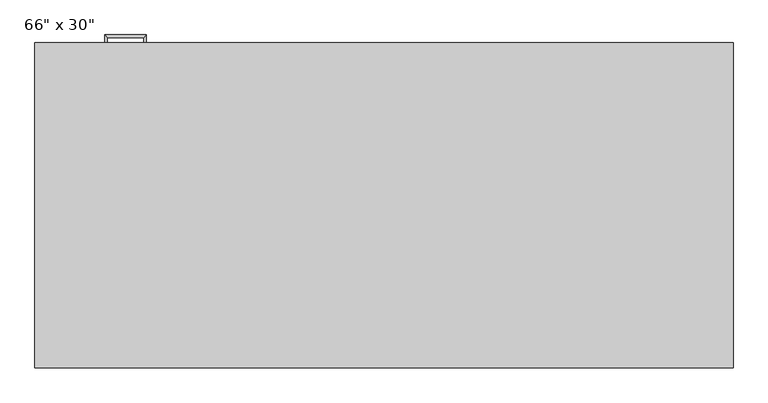
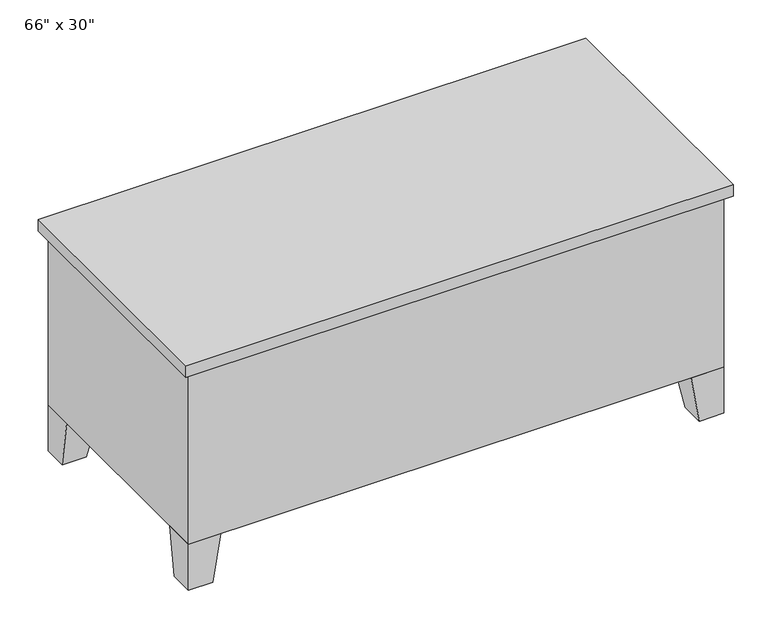
"""IFC4 building model written with IfcOpenShell, lengths in millimetres: furniture geometry."""

import ifcopenshell
import ifcopenshell.guid

model = None  # the IFC model being written
_history = None  # IfcOwnerHistory: only IFC2X3 demands one
_inside = {}  # id of a spatial element -> (the spatial element, [elements in it])
_under = {}  # id of a project, library or spatial element -> (it, [spatial elements below it])
_declared = {}  # id of a project -> (the project, [libraries it declares])
_typed = {}  # id of a type object -> (the type object, [elements of that type])
_made_of = {}  # id of a material, layer set ... -> (it, [elements and type objects made of it])


def new_model(schema):
    """Start an empty IFC model of exactly this schema.

    Asked for "IFC4X3", IfcOpenShell would pick the latest addendum, in which some entities
    have other attributes; the version numbers below select the first issue.
    IFC2X3 requires an IfcOwnerHistory on every rooted entity: one is made here for all.
    """
    global model, _history
    if schema == "IFC4X3":
        model = ifcopenshell.file(schema_version=(4, 3, 0, 0))
    else:
        model = ifcopenshell.file(schema=schema)
    _inside.clear()
    _under.clear()
    _declared.clear()
    _typed.clear()
    _made_of.clear()
    _history = None
    if model.schema == "IFC2X3":
        org = make("IfcOrganization", Name="unknown")
        user = make(
            "IfcPersonAndOrganization",
            ThePerson=make("IfcPerson", FamilyName="unknown"),
            TheOrganization=org,
        )
        app = make(
            "IfcApplication",
            ApplicationDeveloper=org,
            Version="unknown",
            ApplicationFullName="unknown",
            ApplicationIdentifier="unknown",
        )
        _history = make(
            "IfcOwnerHistory",
            OwningUser=user,
            OwningApplication=app,
            ChangeAction="ADDED",
            CreationDate=0,
        )
    return model


def make(cls, **values):
    """One entity of the class cls with the attributes given. An attribute that is None is left unset."""
    return model.create_entity(
        cls, **{name: value for name, value in values.items() if value is not None}
    )


def rooted(cls, **values):
    """An entity with a GlobalId (a new one), such as an element, a storey or a relation."""
    return make(cls, GlobalId=ifcopenshell.guid.new(), OwnerHistory=_history, **values)


def si_unit(unit_type, name, prefix=None):
    """IfcSIUnit, for example si_unit("LENGTHUNIT", "METRE", prefix="MILLI")."""
    return make("IfcSIUnit", UnitType=unit_type, Prefix=prefix, Name=name)


def assignment(units):
    """IfcUnitAssignment: the units of a project."""
    return None if units is None else make("IfcUnitAssignment", Units=units)


def point(xyz):
    """IfcCartesianPoint."""
    return None if xyz is None else make("IfcCartesianPoint", Coordinates=xyz)


def direction(xyz):
    """IfcDirection."""
    return None if xyz is None else make("IfcDirection", DirectionRatios=xyz)


def frame(location, z_axis=None, x_axis=None):
    """IfcAxis2Placement3D, a coordinate frame: its origin and axes. An axis left out is left unset."""
    return make(
        "IfcAxis2Placement3D",
        Location=point(location),
        Axis=direction(z_axis),
        RefDirection=direction(x_axis),
    )


def origin():
    """The frame at (0, 0, 0) with its axes left unset."""
    return frame((0.0, 0.0, 0.0))


def place(relative_to, where):
    """IfcLocalPlacement: puts the frame where relative to a parent placement (None: the world)."""
    return make(
        "IfcLocalPlacement", PlacementRelTo=relative_to, RelativePlacement=where
    )


def context(
    kind, dimensions, precision=None, world=None, true_north=None, identifier=None
):
    """IfcGeometricRepresentationContext, for example the 3D "Model" context."""
    return make(
        "IfcGeometricRepresentationContext",
        ContextIdentifier=identifier,
        ContextType=kind,
        CoordinateSpaceDimension=dimensions,
        Precision=precision,
        WorldCoordinateSystem=world,
        TrueNorth=true_north,
    )


def project(units=None, contexts=None):
    """IfcProject with its units and contexts."""
    return rooted(
        "IfcProject",
        Name="project",
        RepresentationContexts=contexts,
        UnitsInContext=assignment(units),
    )


def spatial(cls, under=None, at=None, **own):
    """A site, building, storey or space (cls), placed at a placement, below another one or the project."""
    s = rooted(cls, ObjectPlacement=at, **own)
    if under is not None:
        _under.setdefault(under.id(), (under, []))[1].append(s)
    return s


def polyline(points):
    """IfcPolyline through the points."""
    return make("IfcPolyline", Points=[point(p) for p in points])


def outline(outer, holes=None, kind="AREA"):
    """IfcArbitraryClosedProfileDef: a profile drawn as a closed curve; with holes, ...WithVoids."""
    if holes is None:
        return make("IfcArbitraryClosedProfileDef", ProfileType=kind, OuterCurve=outer)
    return make(
        "IfcArbitraryProfileDefWithVoids",
        ProfileType=kind,
        OuterCurve=outer,
        InnerCurves=holes,
    )


def extrude(swept, where, along, depth):
    """IfcExtrudedAreaSolid: the profile swept, set in the frame where, extruded along a direction by depth."""
    return make(
        "IfcExtrudedAreaSolid",
        SweptArea=swept,
        Position=where,
        ExtrudedDirection=direction(along),
        Depth=depth,
    )


def faces_of(points, faces, orient=None, outer=None):
    """IfcFace entities. A face is a list of loops; a loop is a list of indices into points, from 0.

    orient and outer hold one flag for each loop. By default every Orientation is true, the
    first loop of a face is its IfcFaceOuterBound and the others are IfcFaceBound.
    """
    made = []
    for i, loops in enumerate(faces):
        bounds = []
        for j, loop in enumerate(loops):
            is_outer = j == 0 if outer is None else outer[i][j]
            bounds.append(
                make(
                    "IfcFaceOuterBound" if is_outer else "IfcFaceBound",
                    Bound=make("IfcPolyLoop", Polygon=[points[k] for k in loop]),
                    Orientation=True if orient is None else orient[i][j],
                )
            )
        made.append(make("IfcFace", Bounds=bounds))
    return made


def faceted_brep(points, faces, orient=None, outer=None, voids=None):
    """IfcFacetedBrep: a solid bounded by flat faces; with voids (closed shells), ...WithVoids."""
    shared = [point(p) for p in points]
    hull = make("IfcClosedShell", CfsFaces=faces_of(shared, faces, orient, outer))
    if voids is None:
        return make("IfcFacetedBrep", Outer=hull)
    return make(
        "IfcFacetedBrepWithVoids",
        Outer=hull,
        Voids=[
            make(cls, CfsFaces=faces_of(shared, fs, o, b)) for cls, fs, o, b in voids
        ],
    )


def shape(context_of_items, identifier, shape_type, items):
    """IfcShapeRepresentation: the items that make up one representation, for example the "Body"."""
    return make(
        "IfcShapeRepresentation",
        ContextOfItems=context_of_items,
        RepresentationIdentifier=identifier,
        RepresentationType=shape_type,
        Items=items,
    )


def source(mapping_origin, context_of_items, identifier, shape_type, items):
    """IfcRepresentationMap: a shape defined once, which mapped items show again and again."""
    return make(
        "IfcRepresentationMap",
        MappingOrigin=mapping_origin,
        MappedRepresentation=shape(context_of_items, identifier, shape_type, items),
    )


def transform(
    local_origin,
    x_axis=None,
    y_axis=None,
    z_axis=None,
    scale=None,
    scale2=None,
    scale3=None,
    uniform=True,
):
    """IfcCartesianTransformationOperator3D, or its non-uniform kind. x_axis, y_axis, z_axis: its Axis1, 2, 3."""
    if uniform:
        return make(
            "IfcCartesianTransformationOperator3D",
            Axis1=direction(x_axis),
            Axis2=direction(y_axis),
            LocalOrigin=point(local_origin),
            Scale=scale,
            Axis3=direction(z_axis),
        )
    return make(
        "IfcCartesianTransformationOperator3DnonUniform",
        Axis1=direction(x_axis),
        Axis2=direction(y_axis),
        LocalOrigin=point(local_origin),
        Scale=scale,
        Axis3=direction(z_axis),
        Scale2=scale2,
        Scale3=scale3,
    )


def mapped(mapping_source, mapping_target):
    """IfcMappedItem: shows the shape of a source again, moved by a transform."""
    return make(
        "IfcMappedItem", MappingSource=mapping_source, MappingTarget=mapping_target
    )


def made_of(thing, what):
    """Note that an element or type object is made of a material, layer set ...; save() writes the relation."""
    if what is not None:
        _made_of.setdefault(what.id(), (what, []))[1].append(thing)
    return thing


def element(
    cls,
    number,
    at=None,
    inside=None,
    cuts=None,
    type_object=None,
    material=None,
    context=None,
    identifier="Body",
    shape_type=None,
    held_by="IfcProductDefinitionShape",
    body=None,
    shapes=None,
    **own,
):
    """One element of the class cls, such as IfcWall. Its Tag is "e" and its number.

    at: its placement. inside: the storey or other place that contains it. cuts: it is an
    opening in that element (IfcRelVoidsElement). A single representation is given by context,
    identifier, shape_type and body (its items); several are given by shapes. held_by: the class
    of the entity that holds the representations. save() writes the other relations.
    """
    e = rooted(cls, Tag="e%d" % number, ObjectPlacement=at, **own)
    if body is not None:
        shapes = [shape(context, identifier, shape_type, body)]
    if shapes is not None:
        e.Representation = make(held_by, Representations=shapes)
    if inside is not None:
        _inside.setdefault(inside.id(), (inside, []))[1].append(e)
    if cuts is not None:
        rooted(
            "IfcRelVoidsElement", RelatingBuildingElement=cuts, RelatedOpeningElement=e
        )
    if type_object is not None:
        _typed.setdefault(type_object.id(), (type_object, []))[1].append(e)
    return made_of(e, material)


def aggregate(whole, parts):
    """IfcRelAggregates: a whole, such as a stair, and the parts it consists of."""
    return rooted("IfcRelAggregates", RelatingObject=whole, RelatedObjects=parts)


def save(model, path):
    """Write the relations noted so far, then the file.

    IfcRelAggregates (storeys below a building ...), IfcRelContainedInSpatialStructure (elements
    in a storey), IfcRelDefinesByType, IfcRelAssociatesMaterial and IfcRelDeclares: one each for
    every whole, place, type object, material and project.
    """
    for whole, parts in _under.values():
        aggregate(whole, parts)
    for where, things in _inside.values():
        rooted(
            "IfcRelContainedInSpatialStructure",
            RelatedElements=things,
            RelatingStructure=where,
        )
    for kind, things in _typed.values():
        rooted("IfcRelDefinesByType", RelatedObjects=things, RelatingType=kind)
    for what, things in _made_of.values():
        rooted("IfcRelAssociatesMaterial", RelatedObjects=things, RelatingMaterial=what)
    for by, libraries in _declared.values():
        rooted("IfcRelDeclares", RelatingContext=by, RelatedDefinitions=libraries)
    model.write(path)


def furniture_388a94df(model_context):
    return source(origin(), model_context, "Body", "SolidModel", [
        faceted_brep([(406.4, 762.0, 723.9), (0.0, 762.0, 723.9), (0.0, 0.0, 723.9), (1676.4, 0.0, 723.9), (1676.4, 762.0, 723.9), (1422.4, 762.0, 723.9), (1422.4, 50.8, 723.9), (406.4, 50.8, 723.9), (406.4, 762.0, 152.4), (406.4, 50.8, 152.4), (1422.4, 50.8, 152.4), (1422.4, 762.0, 152.4), (1676.4, 762.0, 152.4), (1676.4, 0.0, 152.4), (0.0, 0.0, 152.4), (0.0, 762.0, 152.4), (1441.45, 762.0, 171.45), (1657.35, 762.0, 171.45), (1657.35, 762.0, 704.85), (1441.45, 762.0, 704.85), (1441.45, 50.8, 171.45), (1441.45, 50.8, 704.85), (1657.35, 50.8, 704.85), (1657.35, 50.8, 171.45)], [[[0, 1, 2, 3, 4, 5, 6, 7]], [[8, 9, 10, 11, 12, 13, 14, 15]], [[1, 0, 8, 15]], [[2, 1, 15, 14]], [[3, 2, 14, 13]], [[4, 3, 13, 12]], [[5, 4, 12, 11], [16, 17, 18, 19]], [[6, 5, 11, 10]], [[7, 6, 10, 9]], [[0, 7, 9, 8]], [[20, 21, 22, 23]], [[20, 23, 17, 16]], [[23, 22, 18, 17]], [[22, 21, 19, 18]], [[21, 20, 16, 19]]]),
        extrude(outline(polyline([(387.35, 762.0), (19.05, 762.0), (19.05, 774.7), (387.35, 774.7), (387.35, 762.0)])), frame((0.0, 0.0, 603.25), z_axis=(0.0, 0.0, 1.0), x_axis=(1.0, 0.0, 0.0)), (0.0, 0.0, 1.0), 101.6),
        extrude(outline(polyline([(387.35, 762.0), (19.05, 762.0), (19.05, 774.7), (387.35, 774.7), (387.35, 762.0)])), frame((0.0, 0.0, 171.45), z_axis=(0.0, 0.0, 1.0), x_axis=(1.0, 0.0, 0.0)), (0.0, 0.0, 1.0), 171.45),
        extrude(outline(polyline([(387.35, 762.0), (19.05, 762.0), (19.05, 774.7), (387.35, 774.7), (387.35, 762.0)])), frame((0.0, 0.0, 482.6), z_axis=(0.0, 0.0, 1.0), x_axis=(1.0, 0.0, 0.0)), (0.0, 0.0, 1.0), 101.6),
        extrude(outline(polyline([(387.35, 762.0), (19.05, 762.0), (19.05, 774.7), (387.35, 774.7), (387.35, 762.0)])), frame((0.0, 0.0, 361.95), z_axis=(0.0, 0.0, 1.0), x_axis=(1.0, 0.0, 0.0)), (0.0, 0.0, 1.0), 101.6),
        faceted_brep([(1574.8, 762.0, 152.4), (1574.8, 660.4, 152.4), (1676.4, 660.4, 152.4), (1676.4, 762.0, 152.4), (1600.2, 762.0, 0.0), (1676.4, 762.0, 0.0), (1676.4, 685.8, 0.0), (1600.2, 685.8, 0.0)], [[[0, 1, 2, 3]], [[4, 5, 6, 7]], [[4, 7, 1, 0]], [[7, 6, 2, 1]], [[6, 5, 3, 2]], [[5, 4, 0, 3]]]),
        faceted_brep([(1574.8, 0.0, 152.4), (1676.4, 0.0, 152.4), (1676.4, 101.6, 152.4), (1574.8, 101.6, 152.4), (1600.2, 0.0, 0.0), (1600.2, 76.2, 0.0), (1676.4, 76.2, 0.0), (1676.4, 0.0, 0.0)], [[[0, 1, 2, 3]], [[4, 5, 6, 7]], [[4, 7, 1, 0]], [[7, 6, 2, 1]], [[6, 5, 3, 2]], [[5, 4, 0, 3]]]),
        faceted_brep([(101.6, 0.0, 152.4), (101.6, 101.6, 152.4), (0.0, 101.6, 152.4), (0.0, 0.0, 152.4), (76.2, 0.0, 0.0), (0.0, 0.0, 0.0), (0.0, 76.2, 0.0), (76.2, 76.2, 0.0)], [[[0, 1, 2, 3]], [[4, 5, 6, 7]], [[4, 7, 1, 0]], [[7, 6, 2, 1]], [[6, 5, 3, 2]], [[5, 4, 0, 3]]]),
        faceted_brep([(101.6, 762.0, 152.4), (0.0, 762.0, 152.4), (0.0, 660.4, 152.4), (101.6, 660.4, 152.4), (76.2, 762.0, 0.0), (76.2, 685.8, 0.0), (0.0, 685.8, 0.0), (0.0, 762.0, 0.0)], [[[0, 1, 2, 3]], [[4, 5, 6, 7]], [[4, 7, 1, 0]], [[7, 6, 2, 1]], [[6, 5, 3, 2]], [[5, 4, 0, 3]]]),
        extrude(outline(polyline([(1695.45, 781.05), (1695.45, -19.05), (-19.05, -19.05), (-19.05, 781.05), (1695.45, 781.05)])), frame((0.0, 0.0, 723.9), z_axis=(0.0, 0.0, 1.0), x_axis=(1.0, 0.0, 0.0)), (0.0, 0.0, 1.0), 38.1),
        faceted_brep([(158.75, 774.7, 304.8), (152.4, 774.7, 304.8), (152.4, 774.7, 292.1), (158.75, 774.7, 292.1), (158.75, 793.75, 304.8), (152.4, 800.1, 304.8), (152.4, 800.1, 292.1), (158.75, 793.75, 292.1), (247.65, 793.75, 304.8), (254.0, 800.1, 304.8), (254.0, 800.1, 292.1), (247.65, 793.75, 292.1), (247.65, 774.7, 304.8), (247.65, 774.7, 292.1), (254.0, 774.7, 292.1), (254.0, 774.7, 304.8)], [[[0, 1, 2, 3]], [[1, 0, 4, 5]], [[2, 1, 5, 6]], [[3, 2, 6, 7]], [[0, 3, 7, 4]], [[5, 4, 8, 9]], [[6, 5, 9, 10]], [[7, 6, 10, 11]], [[4, 7, 11, 8]], [[12, 13, 14, 15]], [[9, 8, 12, 15]], [[10, 9, 15, 14]], [[11, 10, 14, 13]], [[8, 11, 13, 12]]]),
        faceted_brep([(158.75, 774.7, 425.45), (152.4, 774.7, 425.45), (152.4, 774.7, 412.75), (158.75, 774.7, 412.75), (158.75, 793.75, 425.45), (152.4, 800.1, 425.45), (152.4, 800.1, 412.75), (158.75, 793.75, 412.75), (247.65, 793.75, 425.45), (254.0, 800.1, 425.45), (254.0, 800.1, 412.75), (247.65, 793.75, 412.75), (247.65, 774.7, 425.45), (247.65, 774.7, 412.75), (254.0, 774.7, 412.75), (254.0, 774.7, 425.45)], [[[0, 1, 2, 3]], [[1, 0, 4, 5]], [[2, 1, 5, 6]], [[3, 2, 6, 7]], [[0, 3, 7, 4]], [[5, 4, 8, 9]], [[6, 5, 9, 10]], [[7, 6, 10, 11]], [[4, 7, 11, 8]], [[12, 13, 14, 15]], [[9, 8, 12, 15]], [[10, 9, 15, 14]], [[11, 10, 14, 13]], [[8, 11, 13, 12]]]),
        faceted_brep([(158.75, 774.7, 546.1), (152.4, 774.7, 546.1), (152.4, 774.7, 533.4), (158.75, 774.7, 533.4), (158.75, 793.75, 546.1), (152.4, 800.1, 546.1), (152.4, 800.1, 533.4), (158.75, 793.75, 533.4), (247.65, 793.75, 546.1), (254.0, 800.1, 546.1), (254.0, 800.1, 533.4), (247.65, 793.75, 533.4), (247.65, 774.7, 546.1), (247.65, 774.7, 533.4), (254.0, 774.7, 533.4), (254.0, 774.7, 546.1)], [[[0, 1, 2, 3]], [[1, 0, 4, 5]], [[2, 1, 5, 6]], [[3, 2, 6, 7]], [[0, 3, 7, 4]], [[5, 4, 8, 9]], [[6, 5, 9, 10]], [[7, 6, 10, 11]], [[4, 7, 11, 8]], [[12, 13, 14, 15]], [[9, 8, 12, 15]], [[10, 9, 15, 14]], [[11, 10, 14, 13]], [[8, 11, 13, 12]]]),
        faceted_brep([(158.75, 774.7, 666.75), (152.4, 774.7, 666.75), (152.4, 774.7, 654.05), (158.75, 774.7, 654.05), (158.75, 793.75, 666.75), (152.4, 800.1, 666.75), (152.4, 800.1, 654.05), (158.75, 793.75, 654.05), (247.65, 793.75, 666.75), (254.0, 800.1, 666.75), (254.0, 800.1, 654.05), (247.65, 793.75, 654.05), (247.65, 774.7, 666.75), (247.65, 774.7, 654.05), (254.0, 774.7, 654.05), (254.0, 774.7, 666.75)], [[[0, 1, 2, 3]], [[1, 0, 4, 5]], [[2, 1, 5, 6]], [[3, 2, 6, 7]], [[0, 3, 7, 4]], [[5, 4, 8, 9]], [[6, 5, 9, 10]], [[7, 6, 10, 11]], [[4, 7, 11, 8]], [[12, 13, 14, 15]], [[9, 8, 12, 15]], [[10, 9, 15, 14]], [[11, 10, 14, 13]], [[8, 11, 13, 12]]]),
        extrude(outline(polyline([(1422.4, 381.0), (406.4, 381.0), (406.4, 762.0), (1422.4, 762.0), (1422.4, 381.0)])), frame((0.0, 0.0, 635.0), z_axis=(0.0, 0.0, 1.0), x_axis=(1.0, 0.0, 0.0)), (0.0, 0.0, 1.0), 19.05),
    ])


if __name__ == "__main__":
    model = new_model("IFC4")
    model_context = context("Model", 3, world=origin())
    ifc_project = project(units=[si_unit("LENGTHUNIT", "METRE", prefix="MILLI")], contexts=[model_context])
    site = spatial("IfcSite", under=ifc_project)
    building = spatial("IfcBuilding", under=site)
    placement = place(None, origin())
    furniture_shape = furniture_388a94df(model_context)
    element("IfcFurniture", 1, ObjectType="Desk-Secretary : 66\" x 30\"", at=placement, inside=building, context=model_context, shape_type="MappedRepresentation", body=[
        mapped(furniture_shape, transform((0.0, 0.0, 0.0), x_axis=(1.0, 0.0, 0.0), y_axis=(0.0, 1.0, 0.0), z_axis=(0.0, 0.0, 1.0))),
    ])
    save(model, "model.ifc")

# Revit data of these elements
# Type "Desk-Secretary : 66\" x 30\""
#   Assembly Code = "E2020200"
#   Depth = 2' - 6"
#   Height = 2' - 6"
#   Leg Height = 0' - 6"
#   Width = 5' - 6"
#   Body Material = Laminate, Ivory, Matte
#   Handle/Leg Material = Steel, Chrome Plated
#   Top Material = Cherry
#   Default Elevation = 0
# Element 1 (IfcFurniture, "Desk-Secretary : 66\" x 30\"")
#   Materials on its faces: "Steel, Chrome Plated", "Laminate, Ivory, Matte", "Cherry"
# Materials
#   "Laminate, Ivory, Matte": class "Plastic", colour RGB 247 247 239, transparency 0, Description = "Plastic Laminate - Ivory, Matte", Cost = 0
#   "Steel, Chrome Plated": class "Metal", colour RGB 17 17 17, transparency 0, Description = "Chromiuim plated steel", Cost = 0
#   "Cherry": class "Wood", colour RGB 226 177 128, transparency 0, Description = "Prunus Serotina", Cost = 0
